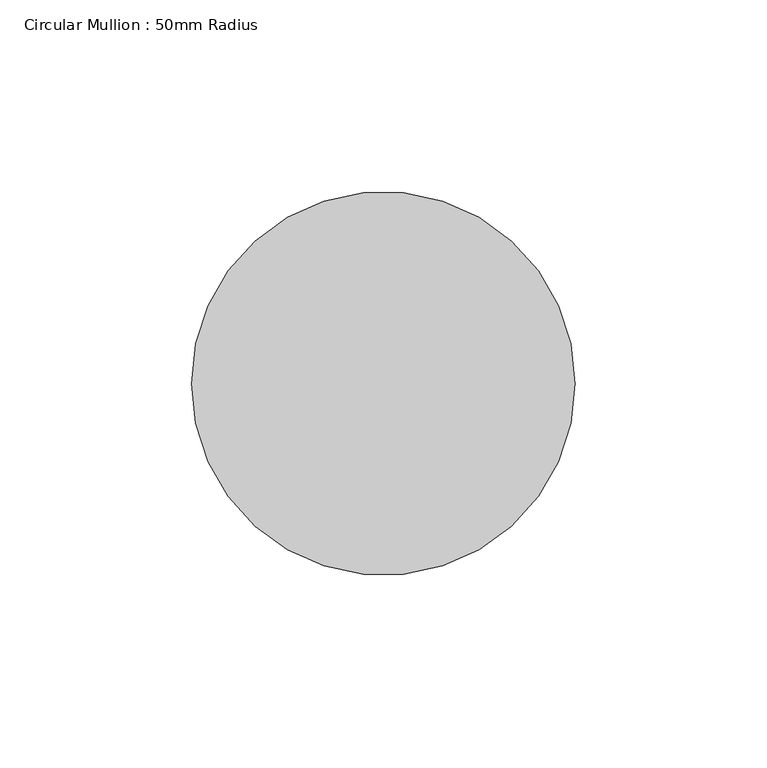
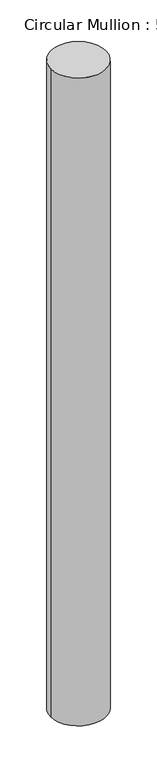
"""IFC4 building model written with IfcOpenShell, lengths in millimetres: member geometry, Circular Mullion : 50mm Radius."""

from ifc_helpers import new_model, si_unit, point, frame, origin, origin_2d, place, context, project, spatial, circle_curve, trimmed, segment, composite_curve, outline, extrude, source, transform, mapped, element, save


def circular_mullion_50mm_radius_67b0ce9a(model_context):
    return source(origin(), model_context, "Body", "SweptSolid", [
        extrude(outline(composite_curve([segment(trimmed(circle_curve(origin_2d(), 50.0), [point((50.0, 0.0))], [point((-50.0, 0.0))], False, "CARTESIAN"), True, "CONTINUOUS"), segment(trimmed(circle_curve(origin_2d(), 50.0), [point((-50.0, 0.0))], [point((50.0, 0.0))], False, "CARTESIAN"), True, "CONTINUOUS")], self_intersect=False)), frame((0.0, 0.0, -1244.3460103), z_axis=(0.0, 0.0, 1.0), x_axis=(1.0, 0.0, 0.0)), (0.0, 0.0, 1.0), 1244.3460103),
    ])


if __name__ == "__main__":
    model = new_model("IFC4")
    model_context = context("Model", 3, world=origin())
    ifc_project = project(units=[si_unit("LENGTHUNIT", "METRE", prefix="MILLI")], contexts=[model_context])
    site = spatial("IfcSite", under=ifc_project)
    building = spatial("IfcBuilding", under=site)
    placement = place(None, origin())
    circular_mullion_50mm_radius_shape = circular_mullion_50mm_radius_67b0ce9a(model_context)
    element("IfcMember", 1, ObjectType="Circular Mullion : 50mm Radius", at=placement, inside=building, context=model_context, shape_type="MappedRepresentation", body=[
        mapped(circular_mullion_50mm_radius_shape, transform((0.0, 0.0, 0.0), x_axis=(1.0, 0.0, 0.0), y_axis=(0.0, 1.0, 0.0), z_axis=(0.0, 0.0, 1.0))),
    ])
    save(model, "model.ifc")

# Revit data of these elements
# Type "Circular Mullion : 50mm Radius"
#   built-in parameter 1007350 = 0.164042 (stored number, unit not read)
# Element 1 (IfcMember, "Circular Mullion : 50mm Radius")
#   Materials on its faces: "Aluminium"
# Materials
#   "Aluminium": class "Metal", colour RGB 247 247 247, transparency 0, Description = "Aluminium 6061", Cost = 0
